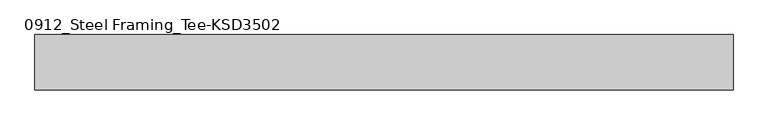
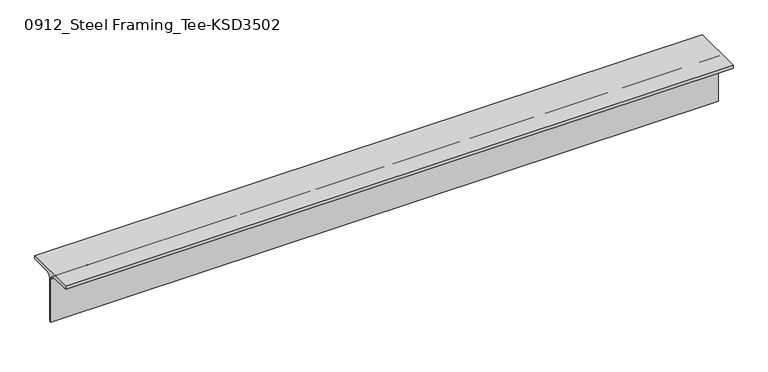
"""IFC4 building model written with IfcOpenShell, lengths in millimetres: member geometry, 0912_Steel Framing_Tee-KSD3502 : H_SB_ASB_CT-150x150x6.5x9."""

from ifc_helpers import new_model, si_unit, point, frame, frame_2d, origin, place, context, project, spatial, polyline, circle_curve, trimmed, segment, composite_curve, outline, extrude, source, transform, mapped, element, save


def member_0912_steel_framing_tee_ksd3502_2efa32de(model_context):
    return source(origin(), model_context, "Body", "SweptSolid", [
        extrude(outline(composite_curve([segment(polyline([(-75.0, 75.0), (75.0, 75.0), (75.0, 66.0), (16.25, 66.0)]), True, "CONTINUOUS"), segment(trimmed(circle_curve(frame_2d((16.25, 53.0)), 13.0), [point((16.25, 66.0))], [point((3.25, 53.0))], True, "CARTESIAN"), True, "CONTINUOUS"), segment(polyline([(3.25, 53.0), (3.25, -75.0), (-3.25, -75.0), (-3.25, 53.0)]), True, "CONTINUOUS"), segment(trimmed(circle_curve(frame_2d((-16.25, 53.0)), 13.0), [point((-3.25, 53.0))], [point((-16.25, 66.0))], True, "CARTESIAN"), True, "CONTINUOUS"), segment(polyline([(-16.25, 66.0), (-75.0, 66.0), (-75.0, 75.0)]), True, "CONTINUOUS")], self_intersect=False)), frame((-900.05, 0.0, 0.0), z_axis=(1.0, 0.0, 0.0), x_axis=(0.0, 1.0, 0.0)), (0.0, 0.0, 1.0), 1884.0),
    ])


if __name__ == "__main__":
    model = new_model("IFC4")
    model_context = context("Model", 3, world=origin())
    ifc_project = project(units=[si_unit("LENGTHUNIT", "METRE", prefix="MILLI")], contexts=[model_context])
    site = spatial("IfcSite", under=ifc_project)
    building = spatial("IfcBuilding", under=site)
    placement = place(None, origin())
    member_0912_steel_framing_tee_ksd3502_shape = member_0912_steel_framing_tee_ksd3502_2efa32de(model_context)
    element("IfcMember", 1, ObjectType="0912_Steel Framing_Tee-KSD3502 : H_SB_ASB_CT-150x150x6.5x9", at=placement, inside=building, context=model_context, shape_type="MappedRepresentation", body=[
        mapped(member_0912_steel_framing_tee_ksd3502_shape, transform((0.0, 0.0, 0.0), x_axis=(1.0, 0.0, 0.0), y_axis=(0.0, 1.0, 0.0), z_axis=(0.0, 0.0, 1.0))),
    ])
    save(model, "model.ifc")

# Revit data of these elements
# Type "0912_Steel Framing_Tee-KSD3502 : H_SB_ASB_CT-150x150x6.5x9"
#   H_WM Code_1 = "S01AA003-00001 | Main Steel Structure Fabrication Work | Shelter/Building | Light Steel - Standard (30KG/M>Weight) | Material: (   )"
#   H_WM Code_2 = "S03AA029-00001 | Main Steel Structure Erection Work | Shelter/Building | Light Steel (30KG/M>Weight) | Material: (   )"
#   H_WM Code_3 = "S01AA010-00001 | Main Steel Structure Fabrication Work | Shelter/Building | Steel Painting/Coating | for Non-Fireproofed Steel Surface, Surface Preparation, Primer, Second & Final Coat | Material: (   )"
#   H_Q'ty Cal Type Tag = "SB-Q2"
#   Width = 15.0 cm
#   Web Thickness = 0.65 cm
#   Web Fillet = 1.3 cm
#   Section Area = 23.39 cm²
#   Perimeter = 0.60 m²/m
#   Nominal Weight = 18.40 kgf/m
#   Height = 15.0 cm
#   Flange Thickness = 0.9 cm
#   Centroid Vertical = 7.5 cm
#   Centroid Horizontal = 7.5 cm
#   Length [instance default] = 1.5000 m
#   Structural Material [instance default] = Steel, 45-345
#   Warping Constant = (empty or 0)
#   Torsional Moment of Inertia = 0
#   Section Name Key = ""
#   Plastic Modulus weak axis = 0
#   Plastic Modulus strong axis = 0
#   Moment of Inertia weak axis = 0
#   Moment of Inertia strong axis = 0
#   Elastic Modulus weak axis = 0
#   Elastic Modulus strong axis = 0
#   Bolt Spacing = 0
#   Assembly Code = ""
# Element 1 (IfcMember, "0912_Steel Framing_Tee-KSD3502 : H_SB_ASB_CT-150x150x6.5x9")
#   Structural Material = none
# Materials
#   "Steel, 45-345": class "Metal", colour RGB 189 187 185, transparency 0, Description = "Steel 345 MPa", Cost = 0
